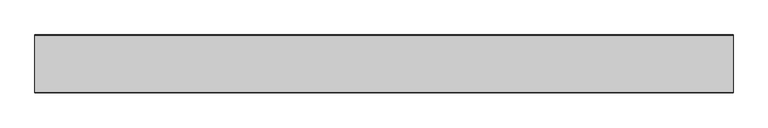
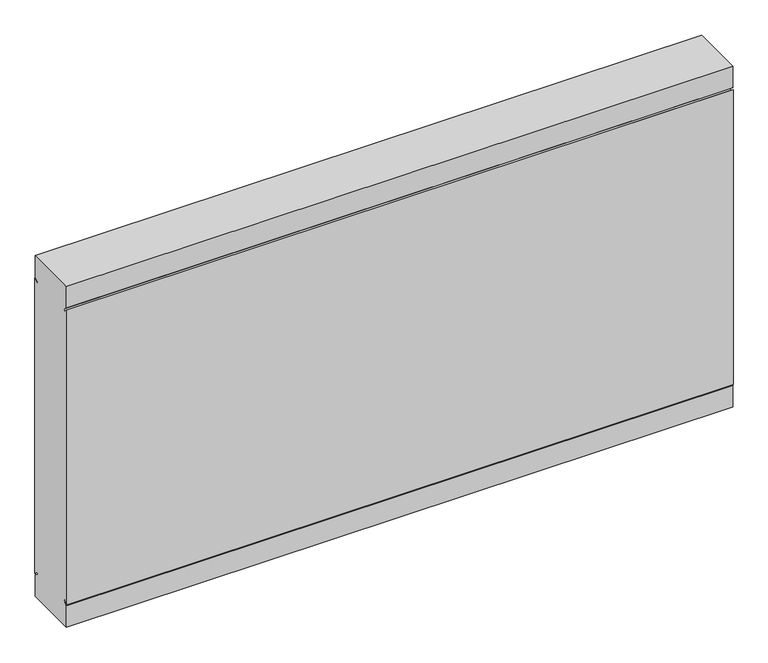
"""IFC4 building model written with IfcOpenShell, lengths in millimetres: proxy geometry, Generic Models 7:Generic Models 1:5:Generic Models 1:5 : Generic Models 7:Generic Models 1:337419:17 : Generic Models 7:Generic Models 1:5:Generic Models 1:5 : Generic Models 7:Generic Models 1:337419:311462."""

from ifc_helpers import new_model, si_unit, frame, origin, place, context, project, spatial, polyline, outline, extrude, source, transform, mapped, element, save


def generic_models_a1b50a28(model_context):
    return source(origin(), model_context, "Body", "SweptSolid", [
        extrude(outline(polyline([(-578799.0788841, 4893.9308169), (-578799.0788841, 3767.0723081), (-578812.2802009, 3778.1495282), (-578816.1067959, 3773.5891699), (-578801.8570091, 3761.632179), (-578801.8570091, 3679.428125), (-578996.3257591, 3679.428125), (-578996.3257591, 3761.632179), (-578982.0759722, 3773.5891699), (-578985.9025672, 3778.1495282), (-578999.1038841, 3767.0723081), (-578999.1038841, 4893.9308169), (-578985.9025672, 4882.8535968), (-578982.0759722, 4887.4139551), (-578996.3257591, 4899.370946), (-578996.3257591, 4981.575), (-578801.8570091, 4981.575), (-578801.8570091, 4899.370946), (-578816.1067959, 4887.4139551), (-578812.2802009, 4882.8535968), (-578799.0788841, 4893.9308169)])), frame((570490.7367239, 0.0, 0.0), z_axis=(1.0, 0.0, 0.0), x_axis=(0.0, 1.0, 0.0)), (0.0, 0.0, 1.0), 2406.65),
    ])


if __name__ == "__main__":
    model = new_model("IFC4")
    model_context = context("Model", 3, world=origin())
    ifc_project = project(units=[si_unit("LENGTHUNIT", "METRE", prefix="MILLI")], contexts=[model_context])
    site = spatial("IfcSite", under=ifc_project)
    building = spatial("IfcBuilding", under=site)
    placement = place(None, origin())
    generic_models_shape = generic_models_a1b50a28(model_context)
    element("IfcBuildingElementProxy", 1, Name="Generic Models 7:Generic Models 1:5:Generic Models 1:5 : Generic Models 7:Generic Models 1:337419:17 : Generic Models 7:Generic Models 1:5:Generic Models 1:5 : Generic Models 7:Generic Models 1:337419:311462", ObjectType="Generic Models 7:Generic Models 1:5:Generic Models 1:5 : Generic Models 7:Generic Models 1:337419:17 : Generic Models 7:Generic Models 1:5:Generic Models 1:5 : Generic Models 7:Generic Models 1:337419:311462", at=placement, inside=building, context=model_context, shape_type="MappedRepresentation", body=[
        mapped(generic_models_shape, transform((0.0, 0.0, 0.0), x_axis=(1.0, 0.0, 0.0), y_axis=(0.0, 1.0, 0.0), z_axis=(0.0, 0.0, 1.0))),
    ])
    save(model, "model.ifc")

# Revit data of these elements
# Type "Generic Models 7:Generic Models 1:5:Generic Models 1:5 : Generic Models 7:Generic Models 1:337419:17 : Generic Models 7:Generic Models 1:5:Generic Models 1:5 : Generic Models 7:Generic Models 1:337419:311462"
#   NameOverride = "Generic Models 7:Generic Models 1:5:Generic Models 1:5 : Generic Models 7:Generic Models 1:337419:311462"
#   ObjectTypeOverride = "Generic Models 1:5 : Generic Models 7:Generic Models 1:337419"
#   Reference = "Generic Models 1"
#   Tag = "311462"
